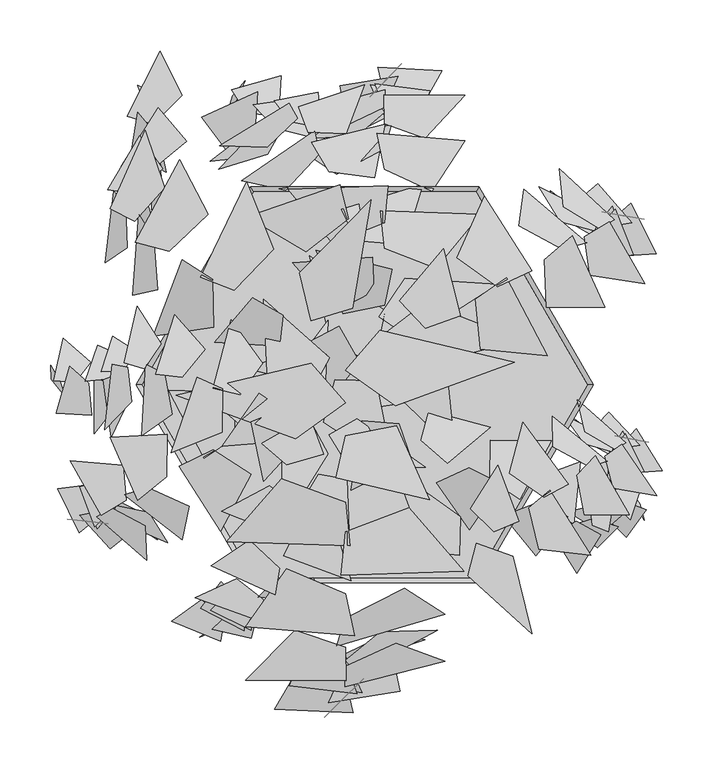
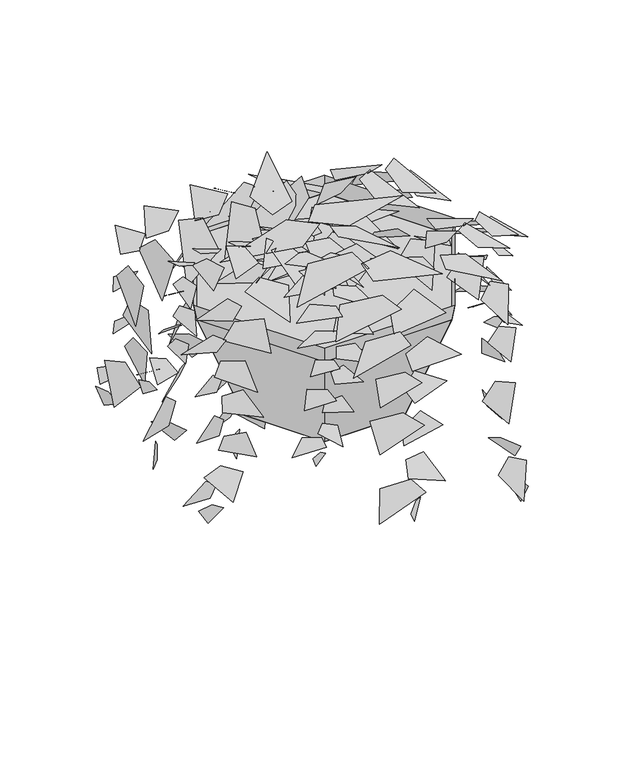
"""IFC4 building model written with IfcOpenShell, lengths in millimetres: geographic element geometry, 吊兰1 3D : 吊兰1 3D."""

from ifc_helpers import new_model, si_unit, origin, place, context, project, spatial, triangles, source, transform, mapped, element, save


def geographic_element_80466ed5(model_context):
    return source(origin(), model_context, "Body", "Tessellation", [
        triangles([(24.2599631, 50.2389166, 267.3885118), (158.8119814, 43.5771957, 241.4721067), (63.9842803, 80.5561385, 262.1539112), (51.8116494, 16.5908296, 259.6649098)], [[2, 1, 3], [1, 2, 4]], closed=False),
        triangles([(24.2599631, 297.8005363, -268.7615384), (29.421192, 303.1911411, -320.0210549), (41.033937, 315.3199611, -277.6829052), (10.0666014, 282.9764229, -285.4699117)], [[2, 1, 3], [1, 2, 4]], closed=False),
        triangles([(24.2599631, 231.9569535, 214.9697455), (-55.0589394, 228.6345546, 153.0443647), (31.5375009, 255.6792337, 179.2892926), (-22.6770247, 206.5734557, 219.6875171)], [[2, 1, 3], [1, 2, 4]], closed=False),
        triangles([(24.2599631, 158.864213, 274.8400918), (-70.1672968, 192.1173976, 216.0915157), (27.7604104, 195.4893939, 266.9692786), (-26.4541175, 138.8656154, 253.3366078)], [[2, 1, 3], [1, 2, 4]], closed=False),
        triangles([(24.2599631, 264.165816, -46.7915162), (67.759595, 285.081963, -116.1540293), (10.9416377, 294.6632277, -58.048578), (59.3281056, 244.126505, -70.2157177)], [[2, 1, 3], [1, 2, 4]], closed=False),
        triangles([(24.2599631, 261.8733869, -98.1583799), (-39.0796095, 249.9470255, -144.0194432), (28.021089, 274.0554195, -130.6746818), (-11.170949, 243.7281827, -88.5725914)], [[2, 1, 3], [1, 2, 4]], closed=False),
        triangles([(24.2599631, 256.3557186, 184.0745019), (103.5788612, 284.2884068, 134.7257154), (23.7592397, 284.5728189, 176.8495614), (64.4201367, 242.1049715, 166.6250947)], [[2, 1, 3], [1, 2, 4]], closed=False),
        triangles([(24.2599631, 272.6144646, -176.3554237), (-19.2396687, 293.5306116, -245.7178687), (37.5782863, 303.1118581, -187.6124401), (-10.808177, 252.5751354, -199.7795935)], [[2, 1, 3], [1, 2, 4]], closed=False),
        triangles([(24.2599631, 267.4978982, 27.8713956), (-49.0186331, 242.2327798, -28.3965589), (15.3293536, 279.018525, -7.0362603), (-3.4487269, 243.3447214, 34.645076)], [[2, 1, 3], [1, 2, 4]], closed=False),
        triangles([(24.2599631, 269.8287879, 80.0999164), (68.9093068, 288.8053731, 27.7385957), (15.09185, 295.8068534, 72.1218514), (55.7527424, 253.3390059, 61.8973392)], [[2, 1, 3], [1, 2, 4]], closed=False),
        triangles([(24.2599631, 284.5377012, -220.1010275), (80.7781181, 308.5586732, -286.3811933), (18.0590539, 311.7768634, -231.558831), (58.7199441, 269.3090341, -241.7832614)], [[2, 1, 3], [1, 2, 4]], closed=False),
        triangles([(24.2599631, 78.0773745, 293.4450608), (-42.655931, 131.9096628, 243.778979), (31.5863215, 113.4699362, 307.6653411), (-16.5243434, 69.6009388, 254.3917215)], [[2, 1, 3], [1, 2, 4]], closed=False),
        triangles([(24.2599631, 134.2455576, 280.5096949), (118.6872231, 167.4987514, 221.7611369), (20.7595137, 170.8707476, 272.6388817), (74.9740392, 114.2469691, 259.0062109)], [[2, 1, 3], [1, 2, 4]], closed=False),
        triangles([(24.2599631, 272.3845186, 137.3668151), (-55.0589394, 268.475255, 75.5038306), (24.7606843, 289.6767225, 106.4353002), (-15.9002104, 253.1376919, 137.3668151)], [[2, 1, 3], [1, 2, 4]], closed=False),
        triangles([(24.2599631, 22.4004632, 241.3319627), (-110.2920597, 15.7387434, 215.4155758), (-15.4643586, 52.7176897, 236.0973621), (-3.291726, -11.2476238, 233.6083607)], [[2, 1, 3], [1, 2, 4]], closed=False),
        triangles([(24.2599631, 211.4250309, 240.9685219), (103.5788612, 239.3577373, 191.6196991), (16.9824243, 246.7201149, 235.447638), (71.1969487, 190.0963182, 221.8149854)], [[2, 1, 3], [1, 2, 4]], closed=False),
        triangles([(117.4295419, 194.4478695, 230.2862161), (-104.3239374, 189.6404413, 201.8188949), (114.6539755, 189.6404413, 201.8188949), (-107.0995129, 194.4478695, 230.2862161), (-104.3239374, -189.6404413, 201.8188949), (-219.3640267, 0.0, 230.2862161), (-107.0995129, -194.4478513, 230.2862161), (-213.8128939, 0.0, 201.8188949), (74.250873, 119.6602288, 0.0), (74.250873, -119.6602197, 0.0), (143.336736, 0.0, 0.0), (-63.920844, -119.6602197, 0.0), (-63.920844, 119.6602288, 0.0), (-133.006707, 0.0, 0.0), (114.6539755, -189.6404413, 201.8188949), (117.4295419, -194.4478513, 230.2862161), (229.6940648, 0.0, 230.2862161), (224.1429501, 0.0, 201.8188949)], [[2, 1, 3], [1, 2, 4], [6, 5, 7], [5, 6, 8], [10, 9, 11], [9, 10, 12], [9, 12, 13], [13, 12, 14], [15, 7, 5], [7, 15, 16], [15, 17, 16], [17, 15, 18], [3, 17, 18], [17, 3, 1], [6, 2, 8], [2, 6, 4], [11, 3, 18], [9, 3, 11], [10, 18, 15], [10, 11, 18], [5, 8, 12], [8, 14, 12], [8, 2, 14], [14, 2, 13], [13, 3, 9], [3, 13, 2], [10, 5, 12], [5, 10, 15]], closed=False),
        triangles([(114.6539755, 189.6404413, 201.8188949), (114.6539755, -189.6404413, 201.8188949), (224.1429501, 0.0, 201.8188949), (-104.3239374, -189.6404413, 201.8188949), (-104.3239374, 189.6404413, 201.8188949), (-213.8128939, 0.0, 201.8188949)], [[2, 1, 3], [1, 2, 4], [1, 4, 5], [5, 4, 6]], closed=False),
        triangles([(38.4629457, -38.2173666, 274.8093161), (-8.3769057, -103.3130525, 243.0681394), (51.1880501, -73.7424056, 267.4729179), (2.3179205, -35.2401682, 266.2751168)], [[2, 1, 3], [1, 2, 4]], closed=False),
        triangles([(270.0535744, -115.8882297, -184.5879699), (275.4567329, -116.9080984, -228.8560527), (279.6633802, -132.6685827, -193.4378657), (263.1453296, -99.6178021, -197.8721154)], [[2, 1, 3], [1, 2, 4]], closed=False),
        triangles([(191.25644, -124.3642385, 229.7241138), (216.7714705, -75.7812937, 182.3309674), (210.3505144, -136.9676571, 198.6269022), (184.91989, -87.469343, 237.1247885)], [[2, 1, 3], [1, 2, 4]], closed=False),
        triangles([(127.8423329, -93.0257081, 281.0728872), (188.2070622, -55.0235582, 237.4334724), (157.3925732, -112.4561718, 274.0445372), (128.4744437, -54.5941649, 266.2815299)], [[2, 1, 3], [1, 2, 4]], closed=False),
        triangles([(231.0691443, -118.0715358, 5.531341), (238.0634485, -145.4132262, -56.9785579), (261.057085, -125.3280605, -3.1957993), (204.578374, -124.4858517, -16.9964462)], [[2, 1, 3], [1, 2, 4]], closed=False),
        triangles([(231.7651048, -112.5413592, -38.4538846), (244.2966073, -69.4276572, -73.2159343), (242.2785255, -117.8139389, -66.5793391), (227.5174353, -85.7119467, -27.7094551)], [[2, 1, 3], [1, 2, 4]], closed=False),
        triangles([(212.9745911, -133.8934534, 203.2407376), (213.4054878, -185.2464326, 155.3182085), (236.8128526, -147.0855715, 197.0587203), (189.3517598, -146.3778203, 185.4615176)], [[2, 1, 3], [1, 2, 4]], closed=False),
        triangles([(244.5832541, -111.2196466, -105.4291207), (279.1493309, -92.8922587, -161.7609112), (266.1294861, -132.4587299, -116.0478766), (240.3200513, -80.8168784, -122.9763054)], [[2, 1, 3], [1, 2, 4]], closed=False),
        triangles([(230.0575782, -126.1097624, 69.4649823), (235.2421818, -70.237814, 26.5112747), (244.1673274, -124.1858973, 40.1936994), (218.5401308, -100.0976601, 77.2593921)], [[2, 1, 3], [1, 2, 4]], closed=False),
        triangles([(229.3499724, -131.7327023, 114.1880791), (233.5199759, -160.1626257, 66.1574898), (254.1230061, -139.1940474, 107.9790377), (206.6619132, -138.4863144, 96.3818077)], [[2, 1, 3], [1, 2, 4]], closed=False),
        triangles([(256.6410391, -113.429786, -142.9033413), (261.9195687, -149.4170244, -203.7015743), (281.6912179, -122.7804598, -152.3042845), (234.2301251, -122.0727269, -163.9015145)], [[2, 1, 3], [1, 2, 4]], closed=False),
        triangles([(60.1514792, -54.3258673, 297.0926034), (128.3434742, -41.8040117, 259.2549784), (86.356811, -77.0366495, 308.7114982), (68.0421495, -25.3541528, 266.554878)], [[2, 1, 3], [1, 2, 4]], closed=False),
        triangles([(107.214495, -81.2324781, 285.954675), (107.7274724, -142.3669551, 228.9040149), (138.983477, -96.9879117, 279.4234603), (75.7020153, -96.0442738, 263.9605233)], [[2, 1, 3], [1, 2, 4]], closed=False),
        triangles([(228.5740932, -137.898069, 163.2254838), (253.6010539, -89.0277781, 115.8864039), (244.2633426, -144.1429459, 136.6832177), (225.3983241, -107.2180377, 166.0982554)], [[2, 1, 3], [1, 2, 4]], closed=False),
        triangles([(16.7744156, -22.1088681, 252.5260468), (55.2189814, 54.0579921, 239.8948956), (54.6783713, -15.9284121, 250.8315827), (-1.9072565, 9.7941026, 247.9049263)], [[2, 1, 3], [1, 2, 4]], closed=False),
        triangles([(172.980339, -116.3452785, 252.0102535), (173.4112538, -167.6982486, 204.0877426), (204.7288008, -129.6553491, 247.7610942), (141.4473437, -128.7117021, 232.2981573)], [[2, 1, 3], [1, 2, 4]], closed=False),
        triangles([(40.2251837, 41.2979425, 281.4703557), (93.7744996, -64.9305434, 262.4798906), (84.3186178, 26.2653822, 277.6346523), (22.9064075, 3.2162593, 275.8108174)], [[2, 1, 3], [1, 2, 4]], closed=False),
        triangles([(257.1128127, 166.5180699, -111.3982149), (264.113421, 165.2991763, -148.95904), (279.8647851, 162.5566838, -117.9354067), (237.8611171, 169.8700092, -123.6414175)], [[2, 1, 3], [1, 2, 4]], closed=False),
        triangles([(199.4275256, 133.2134622, 243.0600549), (161.5087645, 192.1686481, 197.6837185), (223.4225362, 139.6491795, 216.9149211), (156.4731525, 156.2553243, 246.5170386)], [[2, 1, 3], [1, 2, 4]], closed=False),
        triangles([(135.3913089, 96.2421269, 286.9305602), (122.848052, 185.2473955, 243.8820251), (169.0234221, 112.0917318, 281.1631433), (95.4875763, 124.8951745, 271.1737095)], [[2, 1, 3], [1, 2, 4]], closed=False),
        triangles([(227.6455706, 149.5051549, 51.2522359), (265.1690251, 126.8313481, 0.4262923), (248.4860682, 175.1124218, 43.003507), (225.5668094, 112.5609891, 34.0879311)], [[2, 1, 3], [1, 2, 4]], closed=False),
        triangles([(225.6372085, 148.3456236, 13.6127229), (187.2331391, 190.733307, -19.9923798), (237.9698133, 151.6322416, -10.2138728), (194.1025599, 166.2528245, 20.6368081)], [[2, 1, 3], [1, 2, 4]], closed=False),
        triangles([(220.803183, 145.5547056, 220.4213023), (280.28291, 99.0477424, 184.2605553), (245.3030502, 160.2100792, 215.1271668), (226.0431793, 107.6458458, 207.6350914)], [[2, 1, 3], [1, 2, 4]], closed=False),
        triangles([(235.0473899, 153.7785859, -43.686832), (234.1730247, 197.6117752, -94.5127721), (267.6441829, 159.0233421, -51.93552), (202.0134142, 170.4504244, -60.8510959)], [[2, 1, 3], [1, 2, 4]], closed=False),
        triangles([(230.5648147, 151.1905716, 105.9621187), (176.0880527, 194.4292841, 64.7312778), (236.7163651, 163.8449046, 80.3832657), (197.1748651, 160.1555949, 110.9255966)], [[2, 1, 3], [1, 2, 4]], closed=False),
        triangles([(232.6068775, 152.3695604, 144.2330203), (268.9385262, 127.8358017, 105.8648136), (251.3197251, 172.5182306, 138.3870109), (232.0598542, 119.9540154, 130.8949355)], [[2, 1, 3], [1, 2, 4]], closed=False),
        triangles([(245.4932821, 159.8095405, -75.7418158), (291.4827169, 128.7541323, -124.3091638), (266.6205717, 178.3278142, -84.1375969), (247.360719, 125.7635717, -91.6296723)], [[2, 1, 3], [1, 2, 4]], closed=False),
        triangles([(64.6143291, 55.3790234, 300.5635217), (82.2426817, 133.7622931, 264.1702671), (98.8551488, 67.6804119, 310.9835615), (39.1876834, 82.2692698, 271.9468454)], [[2, 1, 3], [1, 2, 4]], closed=False),
        triangles([(113.8230215, 83.7896712, 291.0850123), (184.6322259, 28.4242575, 248.0364953), (144.3652343, 104.9911387, 285.3176136), (118.6854064, 34.9055002, 275.3281434)], [[2, 1, 3], [1, 2, 4]], closed=False),
        triangles([(234.8459487, 153.6622776, 186.1958114), (196.4130112, 212.3206158, 140.8652117), (250.2165585, 162.0261566, 163.5304979), (200.2588702, 174.627604, 186.1958114)], [[2, 1, 3], [1, 2, 4]], closed=False),
        triangles([(15.8360417, 27.2168661, 262.3772079), (-49.3858754, 126.7061741, 243.3867428), (24.86418, 72.9191774, 258.5415045), (-25.8030535, 31.2592043, 256.7176696)], [[2, 1, 3], [1, 2, 4]], closed=False),
        triangles([(181.4396155, 122.8281404, 262.1108724), (240.9193425, 76.3211863, 225.9501254), (209.1494612, 146.2442166, 258.0654071), (183.4696333, 76.1585781, 248.0759733)], [[2, 1, 3], [1, 2, 4]], closed=False),
        triangles([(-13.9299353, -17.8830325, 316.6156669), (-180.0435343, -10.1368483, 300.753045), (-62.9723054, -53.1356193, 313.4117563), (-47.9443619, 21.2426487, 311.8883028)], [[2, 1, 3], [1, 2, 4]], closed=False),
        triangles([(-13.9299353, -305.7454001, -11.5451279), (-20.3018245, -312.0135132, -42.9194733), (-34.638547, -326.1167948, -17.0056287), (3.5927333, -288.508062, -21.7718201)], [[2, 1, 3], [1, 2, 4]], closed=False),
        triangles([(-13.9299353, -229.1830676, 284.5317967), (83.9946278, -225.3198223, 246.6291866), (-22.9145488, -256.7671397, 262.6928863), (44.0169626, -199.667391, 287.4193567)], [[2, 1, 3], [1, 2, 4]], closed=False),
        triangles([(-13.9299353, -144.1915167, 321.176544), (102.6469322, -182.8580246, 285.2183827), (-18.251475, -186.7789517, 316.3590692), (48.6800364, -120.9373311, 308.0149564)], [[2, 1, 3], [1, 2, 4]], closed=False),
        triangles([(-13.9299353, -266.635251, 124.3158221), (-67.6331855, -290.9563683, 81.8612006), (2.5124409, -302.0973307, 117.4257358), (-57.2239326, -243.3337119, 109.978625)], [[2, 1, 3], [1, 2, 4]], closed=False),
        triangles([(-13.9299353, -263.9696434, 92.875799), (64.2670665, -250.1017581, 64.8056464), (-18.5733019, -278.1347853, 72.9735436), (29.8119317, -242.8705497, 98.7429372)], [[2, 1, 3], [1, 2, 4]], closed=False),
        triangles([(-13.9299353, -257.5537378, 265.6217773), (-111.8545007, -290.0335866, 235.4168986), (-13.311759, -290.3643259, 261.199609), (-63.5103948, -240.9830923, 254.9414881)], [[2, 1, 3], [1, 2, 4]], closed=False),
        triangles([(-13.9299353, -276.4592517, 45.0137904), (39.7733127, -300.7803507, 2.5592091), (-30.3723126, -311.9213313, 38.1236995), (29.3640643, -253.1576943, 30.6765909)], [[2, 1, 3], [1, 2, 4]], closed=False),
        triangles([(-13.9299353, -270.5097784, 170.014677), (76.5374703, -241.1317387, 135.5748188), (-2.9044926, -283.9058357, 148.6487846), (20.2783226, -242.4246649, 174.1606449)], [[2, 1, 3], [1, 2, 4]], closed=False),
        triangles([(-13.9299353, -273.2200962, 201.9821661), (-69.0525756, -295.2859005, 169.9333956), (-2.6112789, -303.427155, 197.099034), (-52.8099124, -254.0459395, 190.8408949)], [[2, 1, 3], [1, 2, 4]], closed=False),
        triangles([(-13.9299353, -290.3234672, 18.2384546), (-83.7054285, -318.2548837, -22.3295418), (-6.2744915, -321.9969518, 11.2255287), (-56.4731245, -272.6157181, 4.9674032)], [[2, 1, 3], [1, 2, 4]], closed=False),
        triangles([(-13.9299353, -50.2533279, 332.5640757), (68.6822766, -112.8490075, 302.1650046), (-22.974824, -91.4074838, 341.2678685), (36.42106, -40.3970119, 308.6607382)], [[2, 1, 3], [1, 2, 4]], closed=False),
        triangles([(-13.9299353, -115.5651753, 324.6467537), (-130.5068051, -154.2316651, 288.6885561), (-9.6083956, -158.1526103, 319.8292425), (-76.5399048, -92.3109897, 311.4851297)], [[2, 1, 3], [1, 2, 4]], closed=False),
        triangles([(-13.9299353, -276.1918807, 237.0334242), (83.9946278, -271.6462097, 199.1690203), (-14.5481105, -296.2990836, 218.1012404), (35.6505242, -253.8118332, 237.0334242)], [[2, 1, 3], [1, 2, 4]], closed=False),
        triangles([(-13.9299353, 14.4872618, 300.6672762), (152.1836705, 22.2334471, 284.8046544), (35.1124371, -20.7653273, 297.4633475), (20.0844935, 53.612943, 295.939894)], [[2, 1, 3], [1, 2, 4]], closed=False),
        triangles([(-13.9299353, -205.3087618, 300.4448153), (-111.8545007, -237.7886288, 270.2399365), (-4.9453195, -246.3495343, 297.065661), (-71.8768309, -180.5079319, 288.7215483)], [[2, 1, 3], [1, 2, 4]], closed=False),
        triangles([(-48.5601219, -8.9692711, 288.2841476), (-94.5697999, 84.200193, 272.6449496), (-90.4275927, 2.2078228, 285.125347), (-29.6974855, 26.4383662, 283.6233493)], [[2, 1, 3], [1, 2, 4]], closed=False),
        triangles([(-265.4477509, -134.1893928, -35.2546931), (-272.159169, -133.4714406, -66.1871119), (-287.2598097, -131.8560232, -40.6382717), (-246.9913919, -136.1637908, -45.3373035)], [[2, 1, 3], [1, 2, 4]], closed=False),
        triangles([(-207.7624819, -100.8847941, 256.6521576), (-174.2883442, -152.1416219, 219.2833812), (-231.3496505, -108.0268273, 235.1208411), (-167.4381991, -119.3711567, 259.4990587)], [[2, 1, 3], [1, 2, 4]], closed=False),
        triangles([(-143.7262471, -63.9134589, 292.7807845), (-136.4742279, -143.7540434, 257.3290604), (-177.162224, -80.1027959, 288.0311653), (-106.6642742, -87.6444141, 279.804578)], [[2, 1, 3], [1, 2, 4]], closed=False),
        triangles([(-235.9805088, -117.1764868, 98.6927404), (-271.0664668, -98.7245608, 56.8361066), (-257.5672907, -141.4911364, 91.8997049), (-231.9367149, -83.6358742, 84.557475)], [[2, 1, 3], [1, 2, 4]], closed=False),
        triangles([(-233.9721467, -116.0169464, 67.6955046), (-199.1172974, -152.2571853, 40.0207494), (-246.0940085, -119.6686131, 48.0735918), (-204.422842, -130.4853947, 73.4800398)], [[2, 1, 3], [1, 2, 4]], closed=False),
        triangles([(-229.1381394, -113.2260376, 238.0084737), (-284.1732067, -74.4174144, 208.2290051), (-253.6660572, -127.8328131, 233.6485836), (-232.1277462, -79.2149413, 227.4786295)], [[2, 1, 3], [1, 2, 4]], closed=False),
        triangles([(-243.3823281, -121.4499269, 20.5076713), (-244.9454594, -161.0612082, -21.3490012), (-275.2328186, -127.9873004, 13.7145971), (-212.3134033, -134.7181941, 6.3723684)], [[2, 1, 3], [1, 2, 4]], closed=False),
        triangles([(-238.8997347, -118.8619036, 143.7479845), (-188.5291719, -154.9885048, 109.793153), (-245.5517269, -130.6494744, 122.6830185), (-207.0624701, -125.1376288, 147.835553)], [[2, 1, 3], [1, 2, 4]], closed=False),
        triangles([(-240.9418157, -120.0408923, 175.2651741), (-274.7715458, -99.8405901, 143.6678477), (-260.1683856, -139.2997549, 170.4508059), (-238.6300927, -90.6818922, 164.2808882)], [[2, 1, 3], [1, 2, 4]], closed=False),
        triangles([(-253.8282203, -127.4808724, -5.8905539), (-296.6506428, -101.910867, -45.8871973), (-275.3029814, -145.3972934, -12.8047337), (-253.7646704, -96.7794306, -18.9746969)], [[2, 1, 3], [1, 2, 4]], closed=False),
        triangles([(-72.9492673, -23.0503486, 304.0079335), (-94.3272638, -94.9390633, 274.0370158), (-106.7795561, -36.0628015, 312.5891685), (-49.8079745, -45.9822542, 280.4412761)], [[2, 1, 3], [1, 2, 4]], closed=False),
        triangles([(-122.1579597, -51.4610031, 296.2021055), (-187.6759355, -5.2602746, 260.7503813), (-152.8963178, -72.3227294, 291.4524681), (-124.1785849, -7.4989109, 283.2258808)], [[2, 1, 3], [1, 2, 4]], closed=False),
        triangles([(-243.1808869, -121.3336186, 209.8227668), (-209.1925727, -172.2936077, 172.4916515), (-258.523446, -129.7460685, 191.1572273), (-210.8441616, -138.4011452, 209.8227668)], [[2, 1, 3], [1, 2, 4]], closed=False),
        triangles([(-24.1709788, 5.1118064, 272.5603618), (33.5113062, -81.318483, 256.9211637), (-35.4250724, -36.7350397, 269.4015793), (15.9242551, 3.7435104, 267.8995634)], [[2, 1, 3], [1, 2, 4]], closed=False),
        triangles([(-189.7745537, -90.4994724, 272.3410438), (-244.8096574, -51.6908538, 242.5616115), (-217.892187, -113.2092236, 269.0094884), (-189.1744632, -48.3854005, 260.7829011)], [[2, 1, 3], [1, 2, 4]], closed=False),
        triangles([(-47.7588581, 62.7239557, 295.9149137), (11.4063657, 181.4290057, 318.19613), (-59.0337922, 109.8756062, 303.7119305), (-6.9013093, 74.9248371, 299.2585141)], [[2, 1, 3], [1, 2, 4]], closed=False),
        triangles([(-209.5907679, 271.1982719, -95.0676983), (-206.9955229, 288.4365548, -130.5826907), (-217.8059096, 294.350329, -96.6955967), (-200.0780128, 256.6653836, -111.1972642)], [[2, 1, 3], [1, 2, 4]], closed=False),
        triangles([(-202.57112, 144.6294896, 255.1253976), (-222.8998755, 87.9166086, 186.3889864), (-217.0017436, 167.6029056, 231.1987331), (-198.3048652, 93.2996285, 244.6838293)], [[2, 1, 3], [1, 2, 4]], closed=False),
        triangles([(-144.3964006, 103.5981914, 299.5249768), (-203.0109188, 47.4945846, 227.8960822), (-174.5681418, 122.5598338, 294.3117775), (-143.5319185, 56.5847592, 268.923756)], [[2, 1, 3], [1, 2, 4]], closed=False),
        triangles([(-203.3509234, 211.7833666, 65.6812652), (-198.1403222, 271.8848943, 28.4954968), (-234.0766461, 214.5697699, 53.0142559), (-170.0199092, 239.0477453, 59.7554051)], [[2, 1, 3], [1, 2, 4]], closed=False),
        triangles([(-195.9039216, 221.5972298, 28.6457965), (-204.333567, 171.9392507, -23.502013), (-201.8066681, 236.3744346, 6.1222922), (-194.2160159, 181.9910354, 25.0953977)], [[2, 1, 3], [1, 2, 4]], closed=False),
        triangles([(-220.838101, 160.6005714, 232.4303985), (-210.4751797, 250.1250124, 220.4568016), (-245.1619615, 172.6968171, 226.6046094), (-191.3327435, 193.2665462, 232.2694163)], [[2, 1, 3], [1, 2, 4]], closed=False),
        triangles([(-197.1244503, 242.0955244, -27.9658325), (-224.5988271, 227.2553873, -91.5822733), (-217.8429713, 267.8268571, -32.5405442), (-190.1431359, 208.944114, -55.1993605)], [[2, 1, 3], [1, 2, 4]], closed=False),
        triangles([(-214.1753536, 197.5187031, 119.5132265), (-213.4700006, 136.2589067, 57.0520863), (-224.0101457, 201.603392, 91.4188203), (-203.9878758, 162.804107, 116.3770807)], [[2, 1, 3], [1, 2, 4]], closed=False),
        triangles([(-221.7472933, 187.5402061, 157.1699487), (-216.1885301, 244.3300173, 132.635218), (-247.2722069, 191.4527943, 148.2038535), (-193.4430071, 212.0225417, 153.8686785)], [[2, 1, 3], [1, 2, 4]], closed=False),
        triangles([(-203.0260705, 255.8729356, -59.732237), (-195.9896722, 327.758773, -90.7888897), (-228.1815844, 263.5595304, -70.3287922), (-174.3523664, 284.1292595, -64.6640081)], [[2, 1, 3], [1, 2, 4]], closed=False),
        triangles([(-75.0749324, 68.1649163, 314.267518), (-142.4716453, 41.9041373, 257.2168034), (-105.054407, 85.3350892, 326.1804173), (-78.7938097, 37.8643562, 273.8292523)], [[2, 1, 3], [1, 2, 4]], closed=False),
        triangles([(-123.2716635, 92.8003948, 304.0175623), (-110.9348529, 199.3771108, 289.7632906), (-156.0735948, 105.7314278, 296.677458), (-84.3013224, 133.1577334, 304.2305398)], [[2, 1, 3], [1, 2, 4]], closed=False),
        triangles([(-230.0496572, 176.5991406, 198.4593616), (-249.867143, 119.6440234, 129.7775164), (-241.8538785, 190.2333557, 176.0059719), (-228.1541878, 134.4873488, 186.5718059)], [[2, 1, 3], [1, 2, 4]], closed=False),
        triangles([(-20.4427861, 57.2829952, 277.5623094), (-62.3780557, -55.8196442, 218.088832), (-61.5660186, 35.9971442, 261.2225545), (-0.287187, 22.0175287, 264.1653255)], [[2, 1, 3], [1, 2, 4]], closed=False),
        triangles([(-187.1992022, 131.189585, 274.2235415), (-176.8362991, 220.714017, 262.2499628), (-220.4946263, 139.8575425, 267.4536059), (-148.7223538, 167.283848, 275.0066877)], [[2, 1, 3], [1, 2, 4]], closed=False),
        triangles([(-35.3498772, -68.4408352, 290.8146436), (-131.0758292, -27.3647791, 297.5505878), (-71.6593387, -78.6259057, 295.4211575), (-46.9033962, -37.71774, 289.5760928)], [[2, 1, 3], [1, 2, 4]], closed=False),
        triangles([(-140.3547687, -240.2170598, 80.6183895), (-149.3902546, -242.6058493, 60.2920003), (-157.4141743, -247.7869466, 80.0134391), (-127.8131105, -233.8415769, 71.0601066)], [[2, 1, 3], [1, 2, 4]], closed=False),
        triangles([(-85.8023027, -194.1109169, 278.1413074), (-33.5474663, -213.4092848, 241.7578633), (-99.7993408, -208.5775303, 265.4795985), (-45.6778396, -189.2934966, 272.6113216)], [[2, 1, 3], [1, 2, 4]], closed=False),
        triangles([(-62.4816104, -143.5147865, 299.3404677), (-8.5978315, -192.1895771, 264.1031382), (-74.9219576, -167.8905697, 298.3684158), (-23.0993667, -143.4763986, 282.6938275)], [[2, 1, 3], [1, 2, 4]], closed=False),
        triangles([(-114.4494458, -216.6956394, 171.0847425), (-156.0423104, -219.4371327, 149.0993203), (-113.6655365, -241.4028341, 166.1719973), (-136.0297965, -193.3592005, 165.0047539)], [[2, 1, 3], [1, 2, 4]], closed=False),
        triangles([(-117.8736372, -215.1742025, 149.6457168), (-73.4999104, -224.1705647, 121.6181035), (-126.1862113, -222.6141372, 137.2544855), (-87.3741998, -212.2324489, 148.0231596)], [[2, 1, 3], [1, 2, 4]], closed=False),
        triangles([(-94.4383944, -211.0135916, 266.535675), (-161.6566479, -208.8628326, 257.9556573), (-101.8462089, -230.6623014, 264.881143), (-120.6397111, -190.2895114, 263.9002436)], [[2, 1, 3], [1, 2, 4]], closed=False),
        triangles([(-126.7170564, -222.694601, 117.72024), (-106.623897, -249.0385417, 84.2075418), (-144.8195942, -240.1754199, 116.3368488), (-98.5679297, -218.3857615, 102.3472775)], [[2, 1, 3], [1, 2, 4]], closed=False),
        triangles([(-109.4723059, -218.907096, 202.2469029), (-55.4605592, -221.3927546, 167.915005), (-108.8038329, -229.3360016, 187.1482242), (-83.1349237, -209.7210288, 200.1796236)], [[2, 1, 3], [1, 2, 4]], closed=False),
        triangles([(-105.9906871, -220.4540764, 224.045536), (-146.5769997, -221.5221072, 209.1733515), (-106.7405141, -240.9074791, 220.817935), (-125.5340072, -200.5346891, 219.8370719)], [[2, 1, 3], [1, 2, 4]], closed=False),
        triangles([(-133.1732303, -230.9898432, 100.1560141), (-184.5483102, -232.3417956, 81.33041), (-136.6202492, -251.5142263, 95.9400469), (-155.4137514, -211.1414363, 94.9591384)], [[2, 1, 3], [1, 2, 4]], closed=False),
        triangles([(-40.4185858, -87.6510997, 303.0239456), (-10.582916, -143.075551, 276.231504), (-53.5330424, -110.1097943, 311.6680764), (-12.3863022, -92.9046217, 280.983594)], [[2, 1, 3], [1, 2, 4]], closed=False),
        triangles([(-55.7582154, -126.4911163, 300.4629646), (-135.7799389, -123.9306803, 290.2486171), (-63.2346486, -152.7662022, 298.5632986), (-88.2926394, -98.9358034, 297.2554387)], [[2, 1, 3], [1, 2, 4]], closed=False),
        triangles([(-102.1731966, -222.1502665, 247.9470931), (-49.7637639, -241.0429178, 211.5601789), (-109.3540628, -234.0050117, 236.0373367), (-68.7876027, -219.7418561, 241.6633741)], [[2, 1, 3], [1, 2, 4]], closed=False),
        triangles([(-30.2811663, -49.2305751, 278.6053598), (64.7985475, -81.160989, 249.6853045), (-10.2583185, -80.9696307, 272.685009), (-2.764155, -33.4567287, 270.0656558)], [[2, 1, 3], [1, 2, 4]], closed=False),
        triangles([(-78.5349138, -179.8870759, 287.9076263), (-145.7531583, -177.7363169, 279.3275904), (-82.8104795, -206.2645719, 286.4165473), (-107.8684703, -152.4341912, 285.1087056)], [[2, 1, 3], [1, 2, 4]], closed=False),
        triangles([(18.8485475, 66.6858369, 261.3560311), (135.2422446, 98.6711302, 220.0388402), (44.3797947, 104.746577, 252.2442508), (51.5141521, 44.6177435, 249.809225)], [[2, 1, 3], [1, 2, 4]], closed=False),
        triangles([(-121.2122416, 278.3727613, -225.6757599), (-124.9021962, 283.895462, -273.3895626), (-112.6432788, 298.5273451, -235.5763729), (-131.6261863, 260.979528, -239.6321028)], [[2, 1, 3], [1, 2, 4]], closed=False),
        triangles([(-39.4748207, 226.8430578, 217.9417116), (-116.1030149, 200.4889615, 171.0235544), (-44.4730803, 249.4158988, 184.788866), (-72.790656, 191.0931687, 227.6354695)], [[2, 1, 3], [1, 2, 4]], closed=False),
        triangles([(-10.9574128, 162.9653616, 271.1146651), (-110.7715726, 164.7447043, 230.0372851), (-19.294262, 196.2776633, 264.3955622), (-52.5276395, 130.5427222, 257.2950871)], [[2, 1, 3], [1, 2, 4]], closed=False),
        triangles([(-82.7360382, 251.6983539, -22.2040703), (-59.5960807, 281.6115171, -91.0943489), (-104.5137605, 274.757139, -30.0446414), (-49.3883326, 243.5961595, -48.8086396)], [[2, 1, 3], [1, 2, 4]], closed=False),
        triangles([(-88.7850512, 248.950066, -69.5589628), (-146.8804605, 219.7449446, -103.9681179), (-93.1817396, 260.3500606, -99.6548819), (-113.4360629, 222.9475289, -56.6675758)], [[2, 1, 3], [1, 2, 4]], closed=False),
        triangles([(-50.416849, 248.0131682, 190.1472054), (4.7275066, 294.6001684, 135.2711673), (-59.792703, 272.7527555, 184.3122236), (-13.4688136, 246.5670537, 168.5441636)], [[2, 1, 3], [1, 2, 4]], closed=False),
        triangles([(-102.0257583, 257.3661039, -141.2688117), (-155.1089553, 262.5499444, -198.9873998), (-100.4661515, 287.9962837, -152.5298613), (-130.12695, 229.3278444, -158.8670471)], [[2, 1, 3], [1, 2, 4]], closed=False),
        triangles([(-73.9436561, 255.6930592, 46.6274092), (-138.3247599, 211.7072629, 3.5570023), (-89.5844755, 262.8664041, 15.9418537), (-90.4933863, 226.5268162, 55.7777409)], [[2, 1, 3], [1, 2, 4]], closed=False),
        triangles([(-67.7931776, 258.4874381, 94.7766368), (-40.8793089, 287.2479827, 41.3400639), (-84.226654, 278.7704297, 89.3015168), (-37.9027691, 252.5847279, 73.5334885)], [[2, 1, 3], [1, 2, 4]], closed=False),
        triangles([(-111.1087522, 267.310773, -181.2275645), (-77.0405646, 303.7165269, -248.8688391), (-125.7536432, 289.5050579, -190.2538668), (-79.4297629, 263.3193561, -206.0219087)], [[2, 1, 3], [1, 2, 4]], closed=False),
        triangles([(14.3587802, 91.6981274, 286.0891326), (-65.9981154, 119.6449862, 250.3902579), (12.6040101, 125.315643, 299.1852446), (-24.0648987, 72.0540458, 255.1435833)], [[2, 1, 3], [1, 2, 4]], closed=False),
        triangles([(-3.2426587, 141.2476738, 275.6779222), (62.4053796, 196.7083965, 210.3493153), (-17.7132402, 172.5699898, 269.8578014), (44.0519441, 137.6557147, 248.8337395)], [[2, 1, 3], [1, 2, 4]], closed=False),
        triangles([(-61.0493759, 261.5514044, 147.5707799), (-137.503144, 234.6785534, 100.6943806), (-69.5438656, 276.5712725, 119.4889729), (-90.781768, 233.0950926, 152.2143373)], [[2, 1, 3], [1, 2, 4]], closed=False),
        triangles([(23.3383147, 41.6735464, 236.622966), (-96.0396411, -2.8332522, 229.8619869), (-20.7382304, 57.1512218, 237.7133245), (7.7258803, 3.9424695, 232.1521088)], [[2, 1, 3], [1, 2, 4]], closed=False),
        triangles([(-30.266957, 209.0281205, 241.3311633), (24.8773968, 255.6151206, 186.4551161), (-47.3634607, 238.1319945, 238.1241825), (14.4017236, 203.2177375, 217.1001024)], [[2, 1, 3], [1, 2, 4]], closed=False),
        triangles([(114.8801517, -155.7273768, 297.8234636), (169.094784, -244.2542044, 286.8760396), (150.6048697, -168.4626823, 295.6122977), (106.2627544, -187.2555033, 294.5609084)], [[2, 1, 3], [1, 2, 4]], closed=False),
        triangles([(266.0881732, -52.9665163, 71.3462992), (271.6163605, -54.0186232, 49.6935919), (284.0547728, -56.385857, 67.5777747), (250.8856673, -50.073229, 64.2884451)], [[2, 1, 3], [1, 2, 4]], closed=False),
        triangles([(225.8716055, -80.2976696, 275.681047), (189.4839646, -31.1199891, 249.5229416), (243.5133157, -75.0893347, 260.6091472), (190.0360567, -60.917162, 277.6738941)], [[2, 1, 3], [1, 2, 4]], closed=False),
        triangles([(181.2273283, -110.637878, 300.9711276), (160.635235, -36.648106, 276.1549098), (205.1138972, -97.6661952, 297.646385), (147.0447219, -86.6146804, 291.8877431)], [[2, 1, 3], [1, 2, 4]], closed=False),
        triangles([(245.5444417, -66.9280187, 165.1094713), (277.1624246, -85.9719599, 135.8098244), (258.4028684, -45.7798728, 160.3543655), (248.4949884, -97.5981397, 155.2147991)], [[2, 1, 3], [1, 2, 4]], closed=False),
        triangles([(244.1442547, -67.8795867, 143.4114316), (209.4231182, -32.4583613, 124.0390585), (253.2141044, -65.2202196, 129.6760963), (217.7138367, -52.8283434, 147.4605849)], [[2, 1, 3], [1, 2, 4]], closed=False),
        triangles([(240.7741116, -70.1699311, 262.630481), (292.1934475, -109.1320832, 241.7848783), (257.7919137, -58.1380892, 259.5785779), (249.4659865, -101.6828468, 255.2596009)], [[2, 1, 3], [1, 2, 4]], closed=False),
        triangles([(250.7047736, -63.4210653, 110.3799086), (244.6375204, -27.0128679, 81.0802526), (275.1013404, -59.2507484, 105.6247937), (223.2745983, -49.3872743, 100.4852364)], [[2, 1, 3], [1, 2, 4]], closed=False),
        triangles([(247.5796373, -65.5449, 196.6481712), (200.4060814, -29.3254788, 172.8798001), (250.7478669, -55.0705303, 181.9026868), (220.8246388, -57.9095512, 199.5094428)], [[2, 1, 3], [1, 2, 4]], closed=False),
        triangles([(249.0033149, -64.5773673, 218.7101785), (279.9346573, -85.1592188, 196.5920337), (260.8991186, -47.9504525, 215.3401444), (252.5731733, -91.4952147, 211.0211493)], [[2, 1, 3], [1, 2, 4]], closed=False),
        triangles([(257.9873777, -58.471817, 91.9011855), (297.1409472, -84.5247916, 63.9035122), (271.9387427, -43.212683, 87.0612466), (263.6127975, -86.7574406, 82.7422878)], [[2, 1, 3], [1, 2, 4]], closed=False),
        triangles([(131.8835924, -144.1718594, 308.8301319), (135.7780041, -79.1752363, 287.8504714), (156.6745392, -134.1504054, 314.83696), (109.0398378, -121.6949974, 292.3334463)], [[2, 1, 3], [1, 2, 4]], closed=False),
        triangles([(166.19051, -120.8568945, 303.3660396), (227.4040338, -167.2403914, 278.5498218), (187.0445241, -103.4229205, 300.041297), (175.9432577, -161.4826033, 294.2826732)], [[2, 1, 3], [1, 2, 4]], closed=False),
        triangles([(250.5643388, -63.5165037, 242.9005079), (213.8182533, -14.5824368, 216.7687454), (261.3431322, -56.6578017, 229.8346085), (221.4124845, -45.9081762, 242.9005079)], [[2, 1, 3], [1, 2, 4]], closed=False),
        triangles([(97.8767201, -167.2829033, 286.8168135), (35.5242851, -84.2865159, 275.8693713), (99.1868872, -129.3787217, 284.6056658), (65.39034, -163.6888822, 283.5542765)], [[2, 1, 3], [1, 2, 4]], closed=False),
        triangles([(213.3309465, -88.8202962, 286.6632982), (264.7502644, -127.7824528, 265.8176774), (231.736382, -69.5309939, 284.3312094), (220.6351519, -127.5906677, 278.5725675)], [[2, 1, 3], [1, 2, 4]], closed=False),
        triangles([(-62.3404581, -30.8654057, 287.9505743), (-31.0890499, 63.2664281, 255.4141336), (-74.6140003, 4.9571681, 284.8787959), (-34.441214, -19.6220604, 274.7541414)], [[2, 1, 3], [1, 2, 4]], closed=False),
        triangles([(-294.1081563, 3.1549179, 115.2024249), (-302.7829901, 5.651079, 94.7323626), (-303.2845947, 19.103912, 112.022014), (-289.2691529, -11.5459954, 108.1478319)], [[2, 1, 3], [1, 2, 4]], closed=False),
        triangles([(-191.321298, 11.0612934, 298.203564), (-214.1622185, -50.0434252, 285.1170444), (-210.020956, 20.3506292, 286.8215734), (-184.042073, -28.780404, 303.0422948)], [[2, 1, 3], [1, 2, 4]], closed=False),
        triangles([(-134.7631677, -3.8752441, 309.6623486), (-185.2644184, -66.7564994, 306.5101064), (-159.6568972, 7.233842, 312.265569), (-135.1200591, -46.4249597, 305.4830252)], [[2, 1, 3], [1, 2, 4]], closed=False),
        triangles([(-244.6331238, 5.9445585, 198.586752), (-257.4570322, 38.9991911, 167.5420082), (-269.5340567, 3.2522738, 201.3955377), (-226.1441361, 25.1641594, 180.2555853)], [[2, 1, 3], [1, 2, 4]], closed=False),
        triangles([(-249.2810959, 2.8297785, 177.5542422), (-260.8282654, -48.0591305, 166.9480946), (-260.5904529, 6.9119157, 166.0030941), (-243.7453328, -26.6968125, 183.8023165)], [[2, 1, 3], [1, 2, 4]], closed=False),
        triangles([(-211.5166132, 15.5049459, 289.9952169), (-218.7082709, 77.1102188, 262.6162558), (-231.5455688, 21.6995907, 292.0327924), (-195.0834593, 40.1129404, 274.2681427)], [[2, 1, 3], [1, 2, 4]], closed=False),
        triangles([(-265.9625995, 1.5754986, 147.9881599), (-298.1068402, -28.1224795, 130.506251), (-284.9482139, 18.0962428, 146.644392), (-263.0490782, -29.7942343, 140.5909643)], [[2, 1, 3], [1, 2, 4]], closed=False),
        triangles([(-237.8771772, 10.4719671, 229.1579965), (-243.8831514, -51.3720051, 213.621681), (-251.8469822, 5.1186119, 218.5107176), (-226.9103139, -15.0966644, 232.0371085)], [[2, 1, 3], [1, 2, 4]], closed=False),
        triangles([(-233.151212, 13.6389965, 250.543319), (-242.3601158, 47.8925845, 225.8156314), (-253.6844972, 12.9957184, 253.2437356), (-217.2223878, 31.409068, 235.4790678)], [[2, 1, 3], [1, 2, 4]], closed=False),
        triangles([(-279.2868771, 2.323205, 132.467205), (-290.9437055, 45.6821771, 101.1662813), (-300.4321343, 3.9562737, 133.524299), (-263.9700249, 22.3696216, 115.7596584)], [[2, 1, 3], [1, 2, 4]], closed=False),
        triangles([(-77.9885718, -22.7482458, 303.2162667), (-135.1755881, -60.2909965, 302.9702607), (-98.5362456, -8.0836374, 313.8860733), (-86.0344106, -56.1842296, 292.423448)], [[2, 1, 3], [1, 2, 4]], closed=False),
        triangles([(-117.4619073, -9.6265268, 307.6980062), (-126.0233942, 63.7130805, 275.1039928), (-143.9103565, -3.5671895, 311.3926208), (-95.2942015, 20.9839413, 287.7064031)], [[2, 1, 3], [1, 2, 4]], closed=False),
        triangles([(-227.9693699, 17.111543, 273.9916516), (-250.4066268, -44.1339022, 260.8290648), (-243.260951, 20.1730215, 264.4660702), (-223.8964172, -16.5726587, 276.9358941)], [[2, 1, 3], [1, 2, 4]], closed=False),
        triangles([(-46.6923444, -38.9825633, 272.6849), (-75.202064, -138.9556081, 282.100786), (-76.6093954, -60.4663401, 281.9988482), (-31.0301508, -67.4853112, 268.0788766)], [[2, 1, 3], [1, 2, 4]], closed=False),
        triangles([(-174.3266776, 7.3218988, 305.1110275), (-181.5183171, 68.9271699, 277.7320483), (-200.4326604, 10.447651, 310.109378), (-151.8165145, 34.9987812, 286.4231602)], [[2, 1, 3], [1, 2, 4]], closed=False),
    ])


if __name__ == "__main__":
    model = new_model("IFC4")
    model_context = context("Model", 3, world=origin())
    ifc_project = project(units=[si_unit("LENGTHUNIT", "METRE", prefix="MILLI")], contexts=[model_context])
    site = spatial("IfcSite", under=ifc_project)
    building = spatial("IfcBuilding", under=site)
    placement = place(None, origin())
    geographic_element_shape = geographic_element_80466ed5(model_context)
    element("IfcGeographicElement", 1, ObjectType="吊兰1 3D : 吊兰1 3D", at=placement, inside=building, context=model_context, shape_type="MappedRepresentation", body=[
        mapped(geographic_element_shape, transform((0.0, 0.0, 0.0), x_axis=(1.0, 0.0, 0.0), y_axis=(0.0, 1.0, 0.0), z_axis=(0.0, 0.0, 1.0))),
    ])
    save(model, "model.ifc")

# Revit data of these elements
# Type "吊兰1 3D : 吊兰1 3D"
#   Height = 1000 mm
